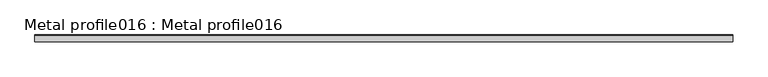
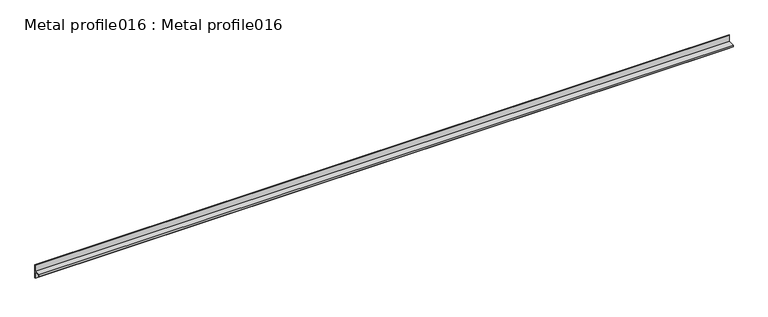
"""IFC4 building model written with IfcOpenShell, lengths in millimetres: proxy geometry, Metal profile016 : Metal profile016."""

from ifc_helpers import new_model, si_unit, frame, origin, place, context, project, spatial, polyline, outline, extrude, source, transform, mapped, element, save


def metal_profile016_metal_profile016_2a48cff6(model_context):
    return source(origin(), model_context, "Body", "SweptSolid", [
        extrude(outline(polyline([(-4439.7287868, 41040.251), (-4439.7287868, 41036.7712), (-4440.9987868, 41036.7712), (-4440.9987868, 41041.521), (-4422.7648388, 41041.521), (-4422.7648388, 41060.571), (-4421.4948388, 41060.571), (-4421.4948388, 41021.201), (-4422.7648388, 41021.201), (-4422.7648388, 41040.251), (-4439.7287868, 41040.251)])), frame((12383.0178845, 0.0, 0.0), z_axis=(1.0, 0.0, 0.0), x_axis=(0.0, 1.0, 0.0)), (0.0, 0.0, 1.0), 2000.0),
    ])


if __name__ == "__main__":
    model = new_model("IFC4")
    model_context = context("Model", 3, world=origin())
    ifc_project = project(units=[si_unit("LENGTHUNIT", "METRE", prefix="MILLI")], contexts=[model_context])
    site = spatial("IfcSite", under=ifc_project)
    building = spatial("IfcBuilding", under=site)
    placement = place(None, origin())
    metal_profile016_metal_profile016_shape = metal_profile016_metal_profile016_2a48cff6(model_context)
    element("IfcBuildingElementProxy", 1, Name="Metal profile016 : Metal profile016", ObjectType="Metal profile016 : Metal profile016", at=placement, inside=building, context=model_context, shape_type="MappedRepresentation", body=[
        mapped(metal_profile016_metal_profile016_shape, transform((0.0, 0.0, 0.0), x_axis=(1.0, 0.0, 0.0), y_axis=(0.0, 1.0, 0.0), z_axis=(0.0, 0.0, 1.0))),
    ])
    save(model, "model.ifc")

# Revit data of these elements
# Type "Metal profile016 : Metal profile016"
#   NameOverride = "Metal profile016"
# Element 1 (IfcBuildingElementProxy, "Metal profile016 : Metal profile016")
#   Materials on its faces: "16 GA. COPPER VENTED T REVEAL BEAD"
# Materials
#   "16 GA. COPPER VENTED T REVEAL BEAD": class "Unassigned", colour RGB 255 227 10, transparency 0
